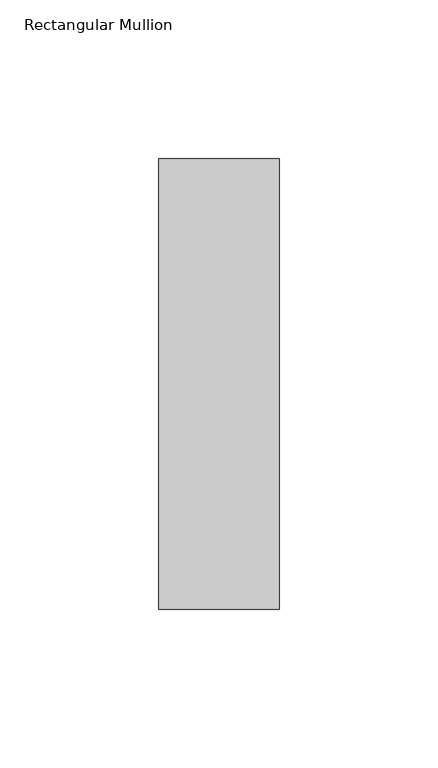
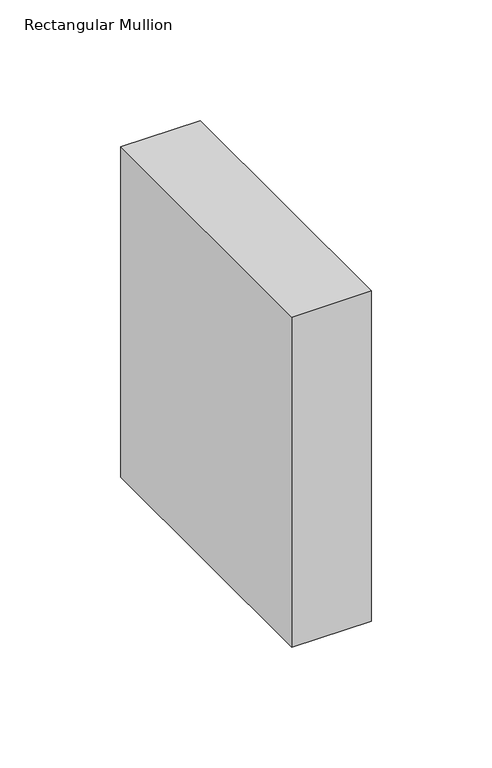
"""IFC4 building model written with IfcOpenShell, lengths in millimetres: member geometry, Rectangular Mullion : NLRS_21_CWM_hsb-regel 38x142_gen_rsf."""

import ifcopenshell
import ifcopenshell.guid

model = None  # the IFC model being written
_history = None  # IfcOwnerHistory: only IFC2X3 demands one
_inside = {}  # id of a spatial element -> (the spatial element, [elements in it])
_under = {}  # id of a project, library or spatial element -> (it, [spatial elements below it])
_declared = {}  # id of a project -> (the project, [libraries it declares])
_typed = {}  # id of a type object -> (the type object, [elements of that type])
_made_of = {}  # id of a material, layer set ... -> (it, [elements and type objects made of it])


def new_model(schema):
    """Start an empty IFC model of exactly this schema.

    Asked for "IFC4X3", IfcOpenShell would pick the latest addendum, in which some entities
    have other attributes; the version numbers below select the first issue.
    IFC2X3 requires an IfcOwnerHistory on every rooted entity: one is made here for all.
    """
    global model, _history
    if schema == "IFC4X3":
        model = ifcopenshell.file(schema_version=(4, 3, 0, 0))
    else:
        model = ifcopenshell.file(schema=schema)
    _inside.clear()
    _under.clear()
    _declared.clear()
    _typed.clear()
    _made_of.clear()
    _history = None
    if model.schema == "IFC2X3":
        org = make("IfcOrganization", Name="unknown")
        user = make(
            "IfcPersonAndOrganization",
            ThePerson=make("IfcPerson", FamilyName="unknown"),
            TheOrganization=org,
        )
        app = make(
            "IfcApplication",
            ApplicationDeveloper=org,
            Version="unknown",
            ApplicationFullName="unknown",
            ApplicationIdentifier="unknown",
        )
        _history = make(
            "IfcOwnerHistory",
            OwningUser=user,
            OwningApplication=app,
            ChangeAction="ADDED",
            CreationDate=0,
        )
    return model


def make(cls, **values):
    """One entity of the class cls with the attributes given. An attribute that is None is left unset."""
    return model.create_entity(
        cls, **{name: value for name, value in values.items() if value is not None}
    )


def rooted(cls, **values):
    """An entity with a GlobalId (a new one), such as an element, a storey or a relation."""
    return make(cls, GlobalId=ifcopenshell.guid.new(), OwnerHistory=_history, **values)


def si_unit(unit_type, name, prefix=None):
    """IfcSIUnit, for example si_unit("LENGTHUNIT", "METRE", prefix="MILLI")."""
    return make("IfcSIUnit", UnitType=unit_type, Prefix=prefix, Name=name)


def assignment(units):
    """IfcUnitAssignment: the units of a project."""
    return None if units is None else make("IfcUnitAssignment", Units=units)


def point(xyz):
    """IfcCartesianPoint."""
    return None if xyz is None else make("IfcCartesianPoint", Coordinates=xyz)


def direction(xyz):
    """IfcDirection."""
    return None if xyz is None else make("IfcDirection", DirectionRatios=xyz)


def frame(location, z_axis=None, x_axis=None):
    """IfcAxis2Placement3D, a coordinate frame: its origin and axes. An axis left out is left unset."""
    return make(
        "IfcAxis2Placement3D",
        Location=point(location),
        Axis=direction(z_axis),
        RefDirection=direction(x_axis),
    )


def origin():
    """The frame at (0, 0, 0) with its axes left unset."""
    return frame((0.0, 0.0, 0.0))


def place(relative_to, where):
    """IfcLocalPlacement: puts the frame where relative to a parent placement (None: the world)."""
    return make(
        "IfcLocalPlacement", PlacementRelTo=relative_to, RelativePlacement=where
    )


def context(
    kind, dimensions, precision=None, world=None, true_north=None, identifier=None
):
    """IfcGeometricRepresentationContext, for example the 3D "Model" context."""
    return make(
        "IfcGeometricRepresentationContext",
        ContextIdentifier=identifier,
        ContextType=kind,
        CoordinateSpaceDimension=dimensions,
        Precision=precision,
        WorldCoordinateSystem=world,
        TrueNorth=true_north,
    )


def project(units=None, contexts=None):
    """IfcProject with its units and contexts."""
    return rooted(
        "IfcProject",
        Name="project",
        RepresentationContexts=contexts,
        UnitsInContext=assignment(units),
    )


def spatial(cls, under=None, at=None, **own):
    """A site, building, storey or space (cls), placed at a placement, below another one or the project."""
    s = rooted(cls, ObjectPlacement=at, **own)
    if under is not None:
        _under.setdefault(under.id(), (under, []))[1].append(s)
    return s


def polyline(points):
    """IfcPolyline through the points."""
    return make("IfcPolyline", Points=[point(p) for p in points])


def outline(outer, holes=None, kind="AREA"):
    """IfcArbitraryClosedProfileDef: a profile drawn as a closed curve; with holes, ...WithVoids."""
    if holes is None:
        return make("IfcArbitraryClosedProfileDef", ProfileType=kind, OuterCurve=outer)
    return make(
        "IfcArbitraryProfileDefWithVoids",
        ProfileType=kind,
        OuterCurve=outer,
        InnerCurves=holes,
    )


def extrude(swept, where, along, depth):
    """IfcExtrudedAreaSolid: the profile swept, set in the frame where, extruded along a direction by depth."""
    return make(
        "IfcExtrudedAreaSolid",
        SweptArea=swept,
        Position=where,
        ExtrudedDirection=direction(along),
        Depth=depth,
    )


def shape(context_of_items, identifier, shape_type, items):
    """IfcShapeRepresentation: the items that make up one representation, for example the "Body"."""
    return make(
        "IfcShapeRepresentation",
        ContextOfItems=context_of_items,
        RepresentationIdentifier=identifier,
        RepresentationType=shape_type,
        Items=items,
    )


def source(mapping_origin, context_of_items, identifier, shape_type, items):
    """IfcRepresentationMap: a shape defined once, which mapped items show again and again."""
    return make(
        "IfcRepresentationMap",
        MappingOrigin=mapping_origin,
        MappedRepresentation=shape(context_of_items, identifier, shape_type, items),
    )


def transform(
    local_origin,
    x_axis=None,
    y_axis=None,
    z_axis=None,
    scale=None,
    scale2=None,
    scale3=None,
    uniform=True,
):
    """IfcCartesianTransformationOperator3D, or its non-uniform kind. x_axis, y_axis, z_axis: its Axis1, 2, 3."""
    if uniform:
        return make(
            "IfcCartesianTransformationOperator3D",
            Axis1=direction(x_axis),
            Axis2=direction(y_axis),
            LocalOrigin=point(local_origin),
            Scale=scale,
            Axis3=direction(z_axis),
        )
    return make(
        "IfcCartesianTransformationOperator3DnonUniform",
        Axis1=direction(x_axis),
        Axis2=direction(y_axis),
        LocalOrigin=point(local_origin),
        Scale=scale,
        Axis3=direction(z_axis),
        Scale2=scale2,
        Scale3=scale3,
    )


def mapped(mapping_source, mapping_target):
    """IfcMappedItem: shows the shape of a source again, moved by a transform."""
    return make(
        "IfcMappedItem", MappingSource=mapping_source, MappingTarget=mapping_target
    )


def made_of(thing, what):
    """Note that an element or type object is made of a material, layer set ...; save() writes the relation."""
    if what is not None:
        _made_of.setdefault(what.id(), (what, []))[1].append(thing)
    return thing


def element(
    cls,
    number,
    at=None,
    inside=None,
    cuts=None,
    type_object=None,
    material=None,
    context=None,
    identifier="Body",
    shape_type=None,
    held_by="IfcProductDefinitionShape",
    body=None,
    shapes=None,
    **own,
):
    """One element of the class cls, such as IfcWall. Its Tag is "e" and its number.

    at: its placement. inside: the storey or other place that contains it. cuts: it is an
    opening in that element (IfcRelVoidsElement). A single representation is given by context,
    identifier, shape_type and body (its items); several are given by shapes. held_by: the class
    of the entity that holds the representations. save() writes the other relations.
    """
    e = rooted(cls, Tag="e%d" % number, ObjectPlacement=at, **own)
    if body is not None:
        shapes = [shape(context, identifier, shape_type, body)]
    if shapes is not None:
        e.Representation = make(held_by, Representations=shapes)
    if inside is not None:
        _inside.setdefault(inside.id(), (inside, []))[1].append(e)
    if cuts is not None:
        rooted(
            "IfcRelVoidsElement", RelatingBuildingElement=cuts, RelatedOpeningElement=e
        )
    if type_object is not None:
        _typed.setdefault(type_object.id(), (type_object, []))[1].append(e)
    return made_of(e, material)


def aggregate(whole, parts):
    """IfcRelAggregates: a whole, such as a stair, and the parts it consists of."""
    return rooted("IfcRelAggregates", RelatingObject=whole, RelatedObjects=parts)


def save(model, path):
    """Write the relations noted so far, then the file.

    IfcRelAggregates (storeys below a building ...), IfcRelContainedInSpatialStructure (elements
    in a storey), IfcRelDefinesByType, IfcRelAssociatesMaterial and IfcRelDeclares: one each for
    every whole, place, type object, material and project.
    """
    for whole, parts in _under.values():
        aggregate(whole, parts)
    for where, things in _inside.values():
        rooted(
            "IfcRelContainedInSpatialStructure",
            RelatedElements=things,
            RelatingStructure=where,
        )
    for kind, things in _typed.values():
        rooted("IfcRelDefinesByType", RelatedObjects=things, RelatingType=kind)
    for what, things in _made_of.values():
        rooted("IfcRelAssociatesMaterial", RelatedObjects=things, RelatingMaterial=what)
    for by, libraries in _declared.values():
        rooted("IfcRelDeclares", RelatingContext=by, RelatedDefinitions=libraries)
    model.write(path)


def rectangular_mullion_f999a466(model_context):
    return source(origin(), model_context, "Body", "SweptSolid", [
        extrude(outline(polyline([(0.0, -71.0), (-38.0, -71.0), (-38.0, 71.0), (0.0, 71.0), (0.0, -71.0)])), frame((0.0, 0.0, -167.1558939), z_axis=(0.0, 0.0, 1.0), x_axis=(1.0, 0.0, 0.0)), (0.0, 0.0, 1.0), 167.1558939),
    ])


if __name__ == "__main__":
    model = new_model("IFC4")
    model_context = context("Model", 3, world=origin())
    ifc_project = project(units=[si_unit("LENGTHUNIT", "METRE", prefix="MILLI")], contexts=[model_context])
    site = spatial("IfcSite", under=ifc_project)
    building = spatial("IfcBuilding", under=site)
    placement = place(None, origin())
    rectangular_mullion_shape = rectangular_mullion_f999a466(model_context)
    element("IfcMember", 1, ObjectType="Rectangular Mullion : NLRS_21_CWM_hsb-regel 38x142_gen_rsf", at=placement, inside=building, context=model_context, shape_type="MappedRepresentation", body=[
        mapped(rectangular_mullion_shape, transform((0.0, 0.0, 0.0), x_axis=(1.0, 0.0, 0.0), y_axis=(0.0, 1.0, 0.0), z_axis=(0.0, 0.0, 1.0))),
    ])
    save(model, "model.ifc")

# Revit data of these elements
# Type "Rectangular Mullion : NLRS_21_CWM_hsb-regel 38x142_gen_rsf"
#   Export Type to IFC As = "IfcWall"
#   Type IfcGUID = "07M7mRoiH1CR8m_RSKIwpF"
#   Assembly Code = "21.10"
#   built-in parameter 1007322 = 0.465879 (stored number, unit not read)
#   built-in parameter 1007321 = 0.062336 (stored number, unit not read)
#   built-in parameter 1007320 = 0.062336 (stored number, unit not read)
# Element 1 (IfcMember, "Rectangular Mullion : NLRS_21_CWM_hsb-regel 38x142_gen_rsf")
#   Materials on its faces: "NLRS_i2_hout naaldhout vuren_gen_rsf"
# Materials
#   "NLRS_i2_hout naaldhout vuren_gen_rsf": class "I - Hout", colour RGB 234 199 147, transparency 0, Keynote = "i2", Manufacturer = "Revit Standards Foundation", URL = "www.revitstandards.org", Description = "hout vuren", Cost = 0
